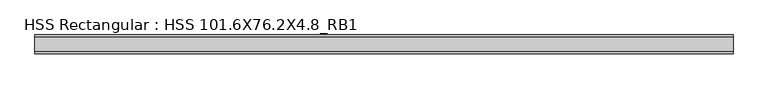
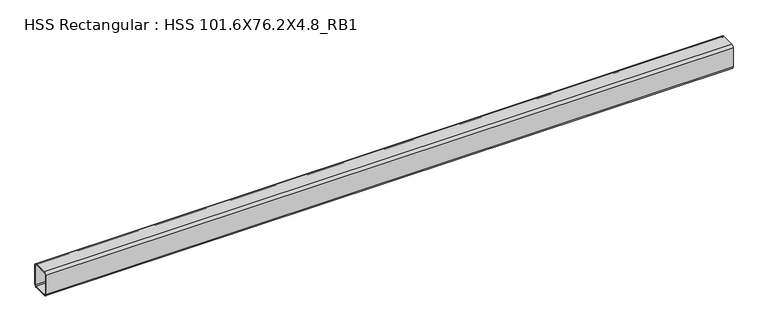
"""IFC4 building model written with IfcOpenShell, lengths in millimetres: beam geometry, HSS Rectangular : HSS 101.6X76.2X4.8_RB1."""

from ifc_helpers import new_model, si_unit, point, frame, frame_2d, origin, place, context, project, spatial, polyline, circle_curve, trimmed, segment, composite_curve, outline, extrude, source, transform, mapped, element, save


def hss_rectangular_hss_101_6x76_2x4_8_rb1_9cb81001(model_context):
    return source(origin(), model_context, "Body", "SweptSolid", [
        extrude(outline(composite_curve([segment(trimmed(circle_curve(frame_2d((-28.575, 41.275)), 9.525), [point((-38.1, 41.275))], [point((-28.575, 50.8))], False, "CARTESIAN"), True, "CONTINUOUS"), segment(polyline([(-28.575, 50.8), (28.575, 50.8)]), True, "CONTINUOUS"), segment(trimmed(circle_curve(frame_2d((28.575, 41.275)), 9.525), [point((28.575, 50.8))], [point((38.1, 41.275))], False, "CARTESIAN"), True, "CONTINUOUS"), segment(polyline([(38.1, 41.275), (38.1, -41.275)]), True, "CONTINUOUS"), segment(trimmed(circle_curve(frame_2d((28.575, -41.275)), 9.525), [point((38.1, -41.275))], [point((28.575, -50.8))], False, "CARTESIAN"), True, "CONTINUOUS"), segment(polyline([(28.575, -50.8), (-28.575, -50.8)]), True, "CONTINUOUS"), segment(trimmed(circle_curve(frame_2d((-28.575, -41.275)), 9.525), [point((-28.575, -50.8))], [point((-38.1, -41.275))], False, "CARTESIAN"), True, "CONTINUOUS"), segment(polyline([(-38.1, -41.275), (-38.1, 41.275)]), True, "CONTINUOUS")], self_intersect=False), holes=[composite_curve([segment(polyline([(28.575, 46.0375), (-28.575, 46.0375)]), True, "CONTINUOUS"), segment(trimmed(circle_curve(frame_2d((-28.575, 41.275)), 4.7625), [point((-28.575, 46.0375))], [point((-33.3375, 41.275))], True, "CARTESIAN"), True, "CONTINUOUS"), segment(polyline([(-33.3375, 41.275), (-33.3375, -41.275)]), True, "CONTINUOUS"), segment(trimmed(circle_curve(frame_2d((-28.575, -41.275)), 4.7625), [point((-33.3375, -41.275))], [point((-28.575, -46.0375))], True, "CARTESIAN"), True, "CONTINUOUS"), segment(polyline([(-28.575, -46.0375), (28.575, -46.0375)]), True, "CONTINUOUS"), segment(trimmed(circle_curve(frame_2d((28.575, -41.275)), 4.7625), [point((28.575, -46.0375))], [point((33.3375, -41.275))], True, "CARTESIAN"), True, "CONTINUOUS"), segment(polyline([(33.3375, -41.275), (33.3375, 41.275)]), True, "CONTINUOUS"), segment(trimmed(circle_curve(frame_2d((28.575, 41.275)), 4.7625), [point((33.3375, 41.275))], [point((28.575, 46.0375))], True, "CARTESIAN"), True, "CONTINUOUS")], self_intersect=False)]), frame((-1402.3433948, 0.0, 0.0), z_axis=(1.0, 0.0, 0.0), x_axis=(0.0, 1.0, 0.0)), (0.0, 0.0, 1.0), 2804.6867896),
    ])


if __name__ == "__main__":
    model = new_model("IFC4")
    model_context = context("Model", 3, world=origin())
    ifc_project = project(units=[si_unit("LENGTHUNIT", "METRE", prefix="MILLI")], contexts=[model_context])
    site = spatial("IfcSite", under=ifc_project)
    building = spatial("IfcBuilding", under=site)
    placement = place(None, origin())
    hss_rectangular_hss_101_6x76_2x4_8_rb1_shape = hss_rectangular_hss_101_6x76_2x4_8_rb1_9cb81001(model_context)
    element("IfcBeam", 1, ObjectType="HSS Rectangular : HSS 101.6X76.2X4.8_RB1", at=placement, inside=building, context=model_context, shape_type="MappedRepresentation", body=[
        mapped(hss_rectangular_hss_101_6x76_2x4_8_rb1_shape, transform((0.0, 0.0, 0.0), x_axis=(1.0, 0.0, 0.0), y_axis=(0.0, 1.0, 0.0), z_axis=(0.0, 0.0, 1.0))),
    ])
    save(model, "model.ifc")

# Revit data of these elements
# Type "HSS Rectangular : HSS 101.6X76.2X4.8_RB1"
#   Section Name Key = "HSS 4X3X3/16"
#   Assembly Code = "B10"
#   Width = 7.62 cm
#   Wall Nominal Thickness = 0.4763 cm
#   Wall Design Thickness = 0.442 cm
#   Torsional Moment of Inertia = 260.561 cm⁴
#   Torsional Modulus = 61.2876 cm³
#   Section Area = 14.4516 cm²
#   Plastic Modulus weak axis = 40.3122 cm³
#   Plastic Modulus strong axis = 49.1612 cm³
#   Perimeter = 0.881482 m²/m
#   Outer Fillet = 0.9525 cm
#   Nominal Weight = 12.1285 kgf/m
#   Moment of Inertia weak axis = 131.529 cm⁴
#   Moment of Inertia strong axis = 205.202 cm⁴
#   Inner Fillet = 0.4763 cm
#   Height = 10.16 cm
#   Elastic Modulus weak axis = 34.4128 cm³
#   Elastic Modulus strong axis = 40.476 cm³
#   Centroid Vertical = 5.08 cm
#   Centroid Horizontal = 3.81 cm
#   Length [instance default] = 1524 mm
#   Structural Material [instance default] = Steel ASTM A500, Grade B, Rectangular and Square
#   Principal Axes Angle = 0
# Element 1 (IfcBeam, "HSS Rectangular : HSS 101.6X76.2X4.8_RB1")
#   Structural Material = Steel ASTM A992
#   Materials on its faces: "Steel ASTM A992"
# Materials
#   "Steel ASTM A500, Grade B, Rectangular and Square": class "Metal", colour RGB 199 199 199, transparency 0, Description = "Carbon steel", Cost = 0
#   "Steel ASTM A992": class "Metal", colour RGB 199 199 199, transparency 0, Description = "Structural steel 50ksi", Cost = 0
